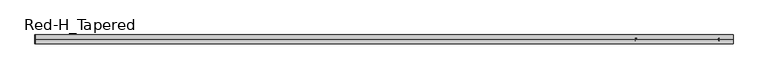
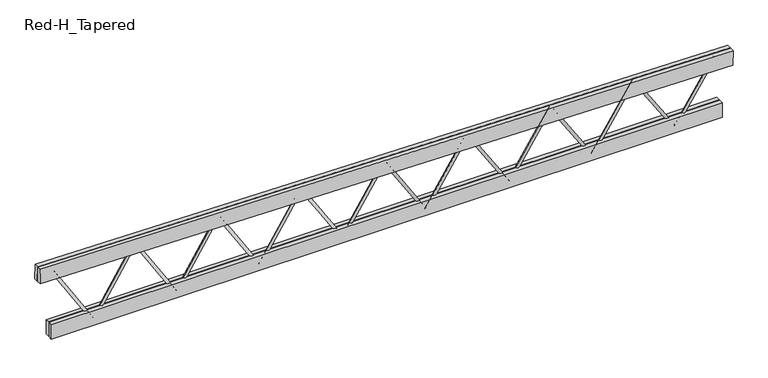
"""IFC4 building model written with IfcOpenShell, lengths in millimetres: beam geometry, Construction_Frames_RedBuilt_Openweb_Red-H_Tapered : Red-H_Tapered."""

from ifc_helpers import new_model, si_unit, point, frame, origin, origin_2d, place, context, project, spatial, polyline, circle_curve, trimmed, segment, composite_curve, outline, extrude, source, transform, mapped, element, save


def red_h_tapered_2e3c5c74(model_context):
    return source(origin(), model_context, "Body", "SweptSolid", [
        extrude(outline(composite_curve([segment(trimmed(circle_curve(origin_2d(), 12.7), [point((0.0, 12.7))], [point((0.0, -12.7))], False, "CARTESIAN"), True, "CONTINUOUS"), segment(trimmed(circle_curve(origin_2d(), 12.7), [point((0.0, -12.7))], [point((0.0, 12.7))], False, "CARTESIAN"), True, "CONTINUOUS")], self_intersect=False)), frame((2671.3982728, 0.0, -367.0101562), z_axis=(0.546899360646311, 0.0, 0.8371983572156938), x_axis=(0.0, -1.0, 0.0)), (0.0, 0.0, 1.0), 697.8035671),
        extrude(outline(composite_curve([segment(trimmed(circle_curve(origin_2d(), 12.7), [point((0.0, -12.7000001))], [point((0.0, 12.6999999))], False, "CARTESIAN"), True, "CONTINUOUS"), segment(trimmed(circle_curve(origin_2d(), 12.7), [point((0.0, 12.6999999))], [point((0.0, -12.7000001))], False, "CARTESIAN"), True, "CONTINUOUS")], self_intersect=False)), frame((2671.3982728, 0.0, -367.0101562), z_axis=(-0.5443057266031581, 0.0, 0.8388869268185123), x_axis=(0.0, -1.0, 0.0)), (0.0, 0.0, 1.0), 701.1286232),
        extrude(outline(composite_curve([segment(trimmed(circle_curve(origin_2d(), 12.7), [point((0.0, 12.7000001))], [point((0.0, -12.7))], False, "CARTESIAN"), True, "CONTINUOUS"), segment(trimmed(circle_curve(origin_2d(), 12.7), [point((0.0, -12.7))], [point((0.0, 12.7000001))], False, "CARTESIAN"), True, "CONTINUOUS")], self_intersect=False)), frame((1908.1416234, 0.0, -367.0101562), z_axis=(0.5443057266031573, 0.0, 0.8388869268185128), x_axis=(0.0, -1.0, 0.0)), (0.0, 0.0, 1.0), 701.1286232),
        extrude(outline(composite_curve([segment(trimmed(circle_curve(origin_2d(), 12.7), [point((0.0, -12.7000001))], [point((0.0, 12.7))], False, "CARTESIAN"), True, "CONTINUOUS"), segment(trimmed(circle_curve(origin_2d(), 12.7), [point((0.0, 12.7))], [point((0.0, -12.7000001))], False, "CARTESIAN"), True, "CONTINUOUS")], self_intersect=False)), frame((1908.1416234, 0.0, -367.0101562), z_axis=(-0.5417314611737056, 0.0, 0.840551618863828), x_axis=(0.0, -1.0, 0.0)), (0.0, 0.0, 1.0), 704.4603314),
        extrude(outline(composite_curve([segment(trimmed(circle_curve(origin_2d(), 12.7), [point((0.0, 12.7000001))], [point((0.0, -12.6999999))], False, "CARTESIAN"), True, "CONTINUOUS"), segment(trimmed(circle_curve(origin_2d(), 12.7), [point((0.0, -12.6999999))], [point((0.0, 12.7000001))], False, "CARTESIAN"), True, "CONTINUOUS")], self_intersect=False)), frame((1144.884974, 0.0, -367.0101562), z_axis=(0.5417314611737046, 0.0, 0.8405516188638286), x_axis=(0.0, -1.0, 0.0)), (0.0, 0.0, 1.0), 704.4603314),
        extrude(outline(composite_curve([segment(trimmed(circle_curve(origin_2d(), 12.7), [point((0.0, -12.7))], [point((0.0, 12.7000001))], False, "CARTESIAN"), True, "CONTINUOUS"), segment(trimmed(circle_curve(origin_2d(), 12.7), [point((0.0, 12.7000001))], [point((0.0, -12.7))], False, "CARTESIAN"), True, "CONTINUOUS")], self_intersect=False)), frame((1144.884974, 0.0, -367.0101562), z_axis=(-0.5391764349852857, 0.0, 0.8421928353747484), x_axis=(0.0, -1.0, 0.0)), (0.0, 0.0, 1.0), 707.7985979),
        extrude(outline(composite_curve([segment(trimmed(circle_curve(origin_2d(), 12.7), [point((0.0, 12.7))], [point((0.0, -12.7))], False, "CARTESIAN"), True, "CONTINUOUS"), segment(trimmed(circle_curve(origin_2d(), 12.7), [point((0.0, -12.7))], [point((0.0, 12.7))], False, "CARTESIAN"), True, "CONTINUOUS")], self_intersect=False)), frame((381.6283247, 0.0, -367.0101562), z_axis=(0.5391764349852862, 0.0, 0.8421928353747482), x_axis=(0.0, -1.0, 0.0)), (0.0, 0.0, 1.0), 707.7985979),
        extrude(outline(composite_curve([segment(trimmed(circle_curve(origin_2d(), 12.7), [point((0.0, -12.7000001))], [point((0.0, 12.6999999))], False, "CARTESIAN"), True, "CONTINUOUS"), segment(trimmed(circle_curve(origin_2d(), 12.7), [point((0.0, 12.6999999))], [point((0.0, -12.7000001))], False, "CARTESIAN"), True, "CONTINUOUS")], self_intersect=False)), frame((381.6283247, 0.0, -367.0101562), z_axis=(-0.5366405174796034, 0.0, 0.843810971129923), x_axis=(0.0, -1.0, 0.0)), (0.0, 0.0, 1.0), 711.1433301),
        extrude(outline(composite_curve([segment(trimmed(circle_curve(origin_2d(), 12.7), [point((0.0, -12.6999999))], [point((0.0, 12.7000001))], False, "CARTESIAN"), True, "CONTINUOUS"), segment(trimmed(circle_curve(origin_2d(), 12.7), [point((0.0, 12.7000001))], [point((0.0, -12.6999999))], False, "CARTESIAN"), True, "CONTINUOUS")], self_intersect=False)), frame((-381.6283247, 0.0, -367.0101562), z_axis=(0.5366405174795735, 0.0, 0.843810971129942), x_axis=(0.0, -1.0, 0.0)), (0.0, 0.0, 1.0), 711.1433301),
        extrude(outline(composite_curve([segment(trimmed(circle_curve(origin_2d(), 12.7), [point((0.0, 12.7))], [point((0.0, -12.7))], False, "CARTESIAN"), True, "CONTINUOUS"), segment(trimmed(circle_curve(origin_2d(), 12.7), [point((0.0, -12.7))], [point((0.0, 12.7))], False, "CARTESIAN"), True, "CONTINUOUS")], self_intersect=False)), frame((-381.6283247, 0.0, -367.0101562), z_axis=(-0.534123577026607, 0.0, 0.8454064137823313), x_axis=(0.0, -1.0, 0.0)), (0.0, 0.0, 1.0), 714.4944374),
        extrude(outline(composite_curve([segment(trimmed(circle_curve(origin_2d(), 12.7), [point((0.0, -12.7))], [point((0.0, 12.7))], False, "CARTESIAN"), True, "CONTINUOUS"), segment(trimmed(circle_curve(origin_2d(), 12.7), [point((0.0, 12.7))], [point((0.0, -12.7))], False, "CARTESIAN"), True, "CONTINUOUS")], self_intersect=False)), frame((-1144.884974, 0.0, -367.0101562), z_axis=(0.5341235770266055, 0.0, 0.8454064137823322), x_axis=(0.0, -1.0, 0.0)), (0.0, 0.0, 1.0), 714.4944374),
        extrude(outline(composite_curve([segment(trimmed(circle_curve(origin_2d(), 12.7), [point((0.0, 12.7))], [point((0.0, -12.7000001))], False, "CARTESIAN"), True, "CONTINUOUS"), segment(trimmed(circle_curve(origin_2d(), 12.7), [point((0.0, -12.7000001))], [point((0.0, 12.7))], False, "CARTESIAN"), True, "CONTINUOUS")], self_intersect=False)), frame((-1144.884974, 0.0, -367.0101562), z_axis=(-0.5316254810336573, 0.0, 0.8469795439771451), x_axis=(0.0, -1.0, 0.0)), (0.0, 0.0, 1.0), 717.8518305),
        extrude(outline(composite_curve([segment(trimmed(circle_curve(origin_2d(), 12.7), [point((0.0, -12.7))], [point((0.0, 12.7))], False, "CARTESIAN"), True, "CONTINUOUS"), segment(trimmed(circle_curve(origin_2d(), 12.7), [point((0.0, 12.7))], [point((0.0, -12.7))], False, "CARTESIAN"), True, "CONTINUOUS")], self_intersect=False)), frame((-1908.1416234, 0.0, -367.0101562), z_axis=(0.5316254810336697, 0.0, 0.8469795439771373), x_axis=(0.0, -1.0, 0.0)), (0.0, 0.0, 1.0), 717.8518305),
        extrude(outline(composite_curve([segment(trimmed(circle_curve(origin_2d(), 12.7), [point((0.0, 12.7))], [point((0.0, -12.7))], False, "CARTESIAN"), True, "CONTINUOUS"), segment(trimmed(circle_curve(origin_2d(), 12.7), [point((0.0, -12.7))], [point((0.0, 12.7))], False, "CARTESIAN"), True, "CONTINUOUS")], self_intersect=False)), frame((-1908.1416234, 0.0, -367.0101562), z_axis=(-0.529146096049623, 0.0, 0.8485307354689299), x_axis=(0.0, -1.0, 0.0)), (0.0, 0.0, 1.0), 721.2154215),
        extrude(outline(composite_curve([segment(trimmed(circle_curve(origin_2d(), 12.7), [point((0.0, -12.7))], [point((0.0, 12.7000001))], False, "CARTESIAN"), True, "CONTINUOUS"), segment(trimmed(circle_curve(origin_2d(), 12.7), [point((0.0, 12.7000001))], [point((0.0, -12.7))], False, "CARTESIAN"), True, "CONTINUOUS")], self_intersect=False)), frame((-2671.3982728, 0.0, -367.0101562), z_axis=(0.529146096049612, 0.0, 0.8485307354689369), x_axis=(0.0, -1.0, 0.0)), (0.0, 0.0, 1.0), 721.2154215),
        extrude(outline(composite_curve([segment(trimmed(circle_curve(origin_2d(), 12.7), [point((0.0, 12.7))], [point((0.0, -12.7))], False, "CARTESIAN"), True, "CONTINUOUS"), segment(trimmed(circle_curve(origin_2d(), 12.7), [point((0.0, -12.7))], [point((0.0, 12.7))], False, "CARTESIAN"), True, "CONTINUOUS")], self_intersect=False)), frame((-2671.3982728, 0.0, -367.0101562), z_axis=(-0.5266852878645721, 0.0, 0.850060355237799), x_axis=(0.0, -1.0, 0.0)), (0.0, 0.0, 1.0), 724.5851241),
        extrude(outline(polyline([(-3078.4265974, -41.275), (-3078.4265974, -3.175), (3078.4265974, -3.175), (3078.4265974, -41.275), (-3078.4265974, -41.275)])), frame((0.0, 0.0, -386.0601562), z_axis=(0.0, 0.0, 1.0), x_axis=(1.0, 0.0, 0.0)), (0.0, 0.0, 1.0), 139.7),
        extrude(outline(polyline([(-3078.4265974, 3.175), (-3078.4265974, 41.275), (3078.4265974, 41.275), (3078.4265974, 3.175), (-3078.4265974, 3.175)])), frame((0.0, 0.0, -386.0601562), z_axis=(0.0, 0.0, 1.0), x_axis=(1.0, 0.0, 0.0)), (0.0, 0.0, 1.0), 139.7),
        extrude(outline(polyline([(0.0, -38.1), (0.0, 0.0), (6360.8646584, 0.0), (6360.8646584, -38.1), (0.0, -38.1)])), frame((-3182.2579796, -3.175, 185.4576655), z_axis=(0.0159726712415793, 0.0, 0.9998724287494922), x_axis=(0.9998724287494922, 0.0, -0.0159726712415793)), (0.0, 0.0, 1.0), 139.7),
        extrude(outline(polyline([(0.0, -38.1), (0.0, 0.0), (6360.8646584, 0.0), (6360.8646584, -38.1), (0.0, -38.1)])), frame((-3182.2579796, 41.275, 185.4576655), z_axis=(0.0159726712415793, 0.0, 0.9998724287494922), x_axis=(0.9998724287494922, 0.0, -0.0159726712415793)), (0.0, 0.0, 1.0), 139.7),
    ])


if __name__ == "__main__":
    model = new_model("IFC4")
    model_context = context("Model", 3, world=origin())
    ifc_project = project(units=[si_unit("LENGTHUNIT", "METRE", prefix="MILLI")], contexts=[model_context])
    site = spatial("IfcSite", under=ifc_project)
    building = spatial("IfcBuilding", under=site)
    placement = place(None, origin())
    red_h_tapered_shape = red_h_tapered_2e3c5c74(model_context)
    element("IfcBeam", 1, ObjectType="Construction_Frames_RedBuilt_Openweb_Red-H_Tapered : Red-H_Tapered", at=placement, inside=building, context=model_context, shape_type="MappedRepresentation", body=[
        mapped(red_h_tapered_shape, transform((0.0, 0.0, 0.0), x_axis=(1.0, 0.0, 0.0), y_axis=(0.0, 1.0, 0.0), z_axis=(0.0, 0.0, 1.0))),
    ])
    save(model, "model.ifc")

# Revit data of these elements
# Type "Construction_Frames_RedBuilt_Openweb_Red-H_Tapered : Red-H_Tapered"
#   Youtube clip = ""
#   Weight Net (Kg) = "0"
#   Webs = "Up to 2\" diameter tubular steel"
#   Uniformat II Description = ""
#   Uniformat II Code = ""
#   Uniclass 2015 Name = "Softwood trusses"
#   Uniclass 2015 Code = "Pr_20_85_90_81"
#   Uniclass 2.0 Description = "Structural Framing Systems"
#   Uniclass 2.0 Code = "SS-15-10-75"
#   Uniclass 1.4 Description = "Trusses"
#   Uniclass 1.4 Code = "L3523"
#   UNSPSC Code = "30103606"
#   Technical description = "http://www.redbuilt.com/reference/literature-and-other-resources"
#   Region South America = "None"
#   Region Oceania = "None"
#   Region North America = "US"
#   Region Middle East = "None"
#   Region Europe = "None"
#   Region Asia = "None"
#   Region Antarctica = "None"
#   Region Africa = "None"
#   QR code = "http://bimobject.com/redbuilt/product/redbuilt-0003"
#   Product url = "http://www.redbuilt.com/products/default.aspx?id=2"
#   Product group = "Wood Trusses"
#   Product family = "Construction"
#   Product data url = "https://bimobject.com/redbuilt/product/redbuilt-0003"
#   Product certification = ""
#   Product SKU = "redbuilt-0003"
#   Product Page URL = "http://www.redbuilt.com/commercial-systems/red-m-red-h-open-web-trusses"
#   Product Guid = "2c5793f2-6ffb-4665-b825-cf90c048e711"
#   Product Documentation Link = "http://www.redbuilt.com/documents/OW_Guide_2017_07_LowRes_wLinks.pdf"
#   OmniClass Description = "Wood Trusses"
#   OmniClass Code = "23-13 35 19 13 17"
#   NBS Reference Description = ""
#   NBS Reference Code = ""
#   Material secondary = "Steel"
#   Material main = "CHARRED WOOD"
#   Masterformat 2014 Description = "Metal-Web Wood Joists"
#   Masterformat 2014 Code = "06 17 36"
#   Manufacturer name = "RedBuilt"
#   Manufacturer country = "United States"
#   Installation instructions = "http://www.redbuilt.com/documents/Installation_Sheets_Open-Web.pdf"
#   IFC Classification = ""
#   EAN code = ""
#   Design country = "United States"
#   Product Information = "http://redbuilt.com/products/default.aspx?id=2"
#   Model = "Red-H-Tapered"
#   Manufacturer URL = "http://redbuilt.com/"
#   Manufacturer = "RedBuilt™"
#   Description = "Open Web Truss"
#   Date of publishing = "8/17/2010"
#   Contact us = "http://redbuilt.com/contact/"
#   Chords = "Double 1½\" x 5½\" MSR lumber"
#   COBIe Type Category = ""
#   Brand url = "http://www.redbuilt.com"
#   BIMobject main category code = "construction"
#   BIMobject main category = "Construction"
#   BIMobject category code = "construction-frames-trusses"
#   BIMobject category = "Frames & Trusses"
#   Web Radius = 0' - 0 1/2"
#   Web Layout Offset Start [instance default] = 0' - 5"
#   Web Layout Offset End [instance default] = 0' - 5"
#   Web Diameter = 0' - 1"
#   TotalLength [instance default] = 20' - 0"
#   Span Minimum = 4' - 0"
#   Span Maximum = 70' - 0"
#   Span Limit [instance default] = 20' - 0"
#   Nominal width = 0' - 0"
#   Nominal height = 0' - 0"
#   Inner Depth Top [instance default] = 0' - 2.76372"
#   Depth Start [instance default] = 6' - 0"
#   Top Chord Length [instance default] = 20' - 1.19701"
#   TC Extension Start Aux [instance default] = 0' - 0"
#   TC Extension End Aux [instance default] = 0' - 0"
#   T-B Chord Length Difference L [instance default] = 0' - 4"
#   T-B Chord Length Difference [instance default] = 0' - 4"
#   Height 2 [instance default] = 6' - 0"
#   Depth Minimum at Wall = 2' - 0"
#   Depth Maximum at Wall = 6' - 0"
#   Depth Lower End [instance default] = 2' - 0"
#   Depth Higher End [instance default] = 6' - 0"
#   Depth End [instance default] = 2' - 0"
#   Depth 2 [instance default] = 2' - 0"
#   Chord Width = 0' - 3 1/4"
#   Chord Thickness = 0' - 1 1/2"
#   Chord Depth = 0' - 5 1/2"
#   Offset Start [instance default] = 0' - 0"
#   TC Extension Start [instance default] = 0' - 0"
#   End Panel = 0' - 5"
#   Offset End [instance default] = 0' - 0"
#   TC Extension End [instance default] = 0' - 0"
#   Length [instance default] = 20' - 0"
#   Angle [instance default] = 5.71059°
#   Span Limit Warning [instance default] = no
#   Edition number = 1
#   Top Bearing Start [instance default] = yes
#   Top Bearing End [instance default] = yes
#   Bottom Bearing Start [instance default] = no
#   Bottom Bearing End [instance default] = no
#   8 Panels [instance default] = yes
#   16 Panels [instance default] = no
#   12 Panels [instance default] = no
#   Web Material = RedBuilt-Steel, Galvanized
#   Clip Material = RedBuilt-Steel, Galvanized
#   Chords Material = OPEN WEB TRUSSES - WOOD TOP/BOTTOM CHORD - TUBE STEEL WEBS
#   URL = ""
#   Assembly Code = ""
# Element 1 (IfcBeam, "Construction_Frames_RedBuilt_Openweb_Red-H_Tapered : Red-H_Tapered")
#   TotalLength = 20' - 10.3958"
#   Span Limit = 20' - 10.3958"
#   Inner Depth Top = 0' - 2.75035"
#   Depth Start = 5' - 0"
#   Top Chord Length = 20' - 10.42774"
#   Height 2 = 5' - 0"
#   Depth Higher End = 5' - 0"
#   Depth 2 = 0' - 4"
#   Angle = 0.915206°
#   Materials on its faces: "RedBuilt-Steel, Galvanized", "OPEN WEB TRUSSES - WOOD TOP/BOTTOM CHORD - TUBE STEEL WEBS"
# Materials
#   "RedBuilt-Steel, Galvanized": class "Metal", colour RGB 164 172 176, transparency 0, Manufacturer = "RedBuilt. LLC", Comments = "Openweb Metal Web", URL = "http://www.redbuilt.com/", Description = "Galvanized steel", Cost = 0
#   "OPEN WEB TRUSSES - WOOD TOP/BOTTOM CHORD - TUBE STEEL WEBS": class "Wood", colour RGB 198 202 183, transparency 0, Description = "Generic wood", Cost = 0
